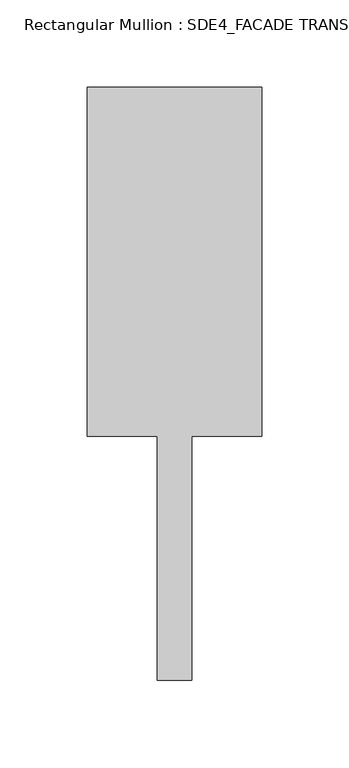
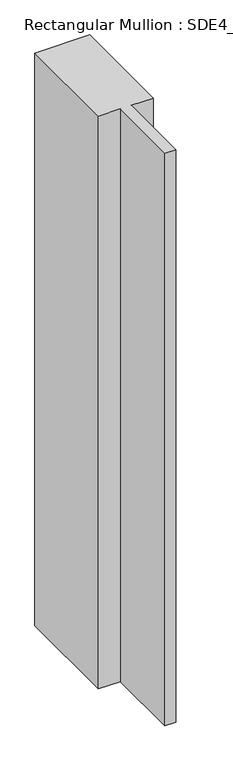
"""IFC4 building model written with IfcOpenShell, lengths in millimetres: member geometry, Rectangular Mullion : SDE4_FACADE TRANSOM TYPE 1."""

import ifcopenshell
import ifcopenshell.guid

model = None  # the IFC model being written
_history = None  # IfcOwnerHistory: only IFC2X3 demands one
_inside = {}  # id of a spatial element -> (the spatial element, [elements in it])
_under = {}  # id of a project, library or spatial element -> (it, [spatial elements below it])
_declared = {}  # id of a project -> (the project, [libraries it declares])
_typed = {}  # id of a type object -> (the type object, [elements of that type])
_made_of = {}  # id of a material, layer set ... -> (it, [elements and type objects made of it])


def new_model(schema):
    """Start an empty IFC model of exactly this schema.

    Asked for "IFC4X3", IfcOpenShell would pick the latest addendum, in which some entities
    have other attributes; the version numbers below select the first issue.
    IFC2X3 requires an IfcOwnerHistory on every rooted entity: one is made here for all.
    """
    global model, _history
    if schema == "IFC4X3":
        model = ifcopenshell.file(schema_version=(4, 3, 0, 0))
    else:
        model = ifcopenshell.file(schema=schema)
    _inside.clear()
    _under.clear()
    _declared.clear()
    _typed.clear()
    _made_of.clear()
    _history = None
    if model.schema == "IFC2X3":
        org = make("IfcOrganization", Name="unknown")
        user = make(
            "IfcPersonAndOrganization",
            ThePerson=make("IfcPerson", FamilyName="unknown"),
            TheOrganization=org,
        )
        app = make(
            "IfcApplication",
            ApplicationDeveloper=org,
            Version="unknown",
            ApplicationFullName="unknown",
            ApplicationIdentifier="unknown",
        )
        _history = make(
            "IfcOwnerHistory",
            OwningUser=user,
            OwningApplication=app,
            ChangeAction="ADDED",
            CreationDate=0,
        )
    return model


def make(cls, **values):
    """One entity of the class cls with the attributes given. An attribute that is None is left unset."""
    return model.create_entity(
        cls, **{name: value for name, value in values.items() if value is not None}
    )


def rooted(cls, **values):
    """An entity with a GlobalId (a new one), such as an element, a storey or a relation."""
    return make(cls, GlobalId=ifcopenshell.guid.new(), OwnerHistory=_history, **values)


def si_unit(unit_type, name, prefix=None):
    """IfcSIUnit, for example si_unit("LENGTHUNIT", "METRE", prefix="MILLI")."""
    return make("IfcSIUnit", UnitType=unit_type, Prefix=prefix, Name=name)


def assignment(units):
    """IfcUnitAssignment: the units of a project."""
    return None if units is None else make("IfcUnitAssignment", Units=units)


def point(xyz):
    """IfcCartesianPoint."""
    return None if xyz is None else make("IfcCartesianPoint", Coordinates=xyz)


def direction(xyz):
    """IfcDirection."""
    return None if xyz is None else make("IfcDirection", DirectionRatios=xyz)


def frame(location, z_axis=None, x_axis=None):
    """IfcAxis2Placement3D, a coordinate frame: its origin and axes. An axis left out is left unset."""
    return make(
        "IfcAxis2Placement3D",
        Location=point(location),
        Axis=direction(z_axis),
        RefDirection=direction(x_axis),
    )


def origin():
    """The frame at (0, 0, 0) with its axes left unset."""
    return frame((0.0, 0.0, 0.0))


def place(relative_to, where):
    """IfcLocalPlacement: puts the frame where relative to a parent placement (None: the world)."""
    return make(
        "IfcLocalPlacement", PlacementRelTo=relative_to, RelativePlacement=where
    )


def context(
    kind, dimensions, precision=None, world=None, true_north=None, identifier=None
):
    """IfcGeometricRepresentationContext, for example the 3D "Model" context."""
    return make(
        "IfcGeometricRepresentationContext",
        ContextIdentifier=identifier,
        ContextType=kind,
        CoordinateSpaceDimension=dimensions,
        Precision=precision,
        WorldCoordinateSystem=world,
        TrueNorth=true_north,
    )


def project(units=None, contexts=None):
    """IfcProject with its units and contexts."""
    return rooted(
        "IfcProject",
        Name="project",
        RepresentationContexts=contexts,
        UnitsInContext=assignment(units),
    )


def spatial(cls, under=None, at=None, **own):
    """A site, building, storey or space (cls), placed at a placement, below another one or the project."""
    s = rooted(cls, ObjectPlacement=at, **own)
    if under is not None:
        _under.setdefault(under.id(), (under, []))[1].append(s)
    return s


def polyline(points):
    """IfcPolyline through the points."""
    return make("IfcPolyline", Points=[point(p) for p in points])


def outline(outer, holes=None, kind="AREA"):
    """IfcArbitraryClosedProfileDef: a profile drawn as a closed curve; with holes, ...WithVoids."""
    if holes is None:
        return make("IfcArbitraryClosedProfileDef", ProfileType=kind, OuterCurve=outer)
    return make(
        "IfcArbitraryProfileDefWithVoids",
        ProfileType=kind,
        OuterCurve=outer,
        InnerCurves=holes,
    )


def extrude(swept, where, along, depth):
    """IfcExtrudedAreaSolid: the profile swept, set in the frame where, extruded along a direction by depth."""
    return make(
        "IfcExtrudedAreaSolid",
        SweptArea=swept,
        Position=where,
        ExtrudedDirection=direction(along),
        Depth=depth,
    )


def shape(context_of_items, identifier, shape_type, items):
    """IfcShapeRepresentation: the items that make up one representation, for example the "Body"."""
    return make(
        "IfcShapeRepresentation",
        ContextOfItems=context_of_items,
        RepresentationIdentifier=identifier,
        RepresentationType=shape_type,
        Items=items,
    )


def source(mapping_origin, context_of_items, identifier, shape_type, items):
    """IfcRepresentationMap: a shape defined once, which mapped items show again and again."""
    return make(
        "IfcRepresentationMap",
        MappingOrigin=mapping_origin,
        MappedRepresentation=shape(context_of_items, identifier, shape_type, items),
    )


def transform(
    local_origin,
    x_axis=None,
    y_axis=None,
    z_axis=None,
    scale=None,
    scale2=None,
    scale3=None,
    uniform=True,
):
    """IfcCartesianTransformationOperator3D, or its non-uniform kind. x_axis, y_axis, z_axis: its Axis1, 2, 3."""
    if uniform:
        return make(
            "IfcCartesianTransformationOperator3D",
            Axis1=direction(x_axis),
            Axis2=direction(y_axis),
            LocalOrigin=point(local_origin),
            Scale=scale,
            Axis3=direction(z_axis),
        )
    return make(
        "IfcCartesianTransformationOperator3DnonUniform",
        Axis1=direction(x_axis),
        Axis2=direction(y_axis),
        LocalOrigin=point(local_origin),
        Scale=scale,
        Axis3=direction(z_axis),
        Scale2=scale2,
        Scale3=scale3,
    )


def mapped(mapping_source, mapping_target):
    """IfcMappedItem: shows the shape of a source again, moved by a transform."""
    return make(
        "IfcMappedItem", MappingSource=mapping_source, MappingTarget=mapping_target
    )


def made_of(thing, what):
    """Note that an element or type object is made of a material, layer set ...; save() writes the relation."""
    if what is not None:
        _made_of.setdefault(what.id(), (what, []))[1].append(thing)
    return thing


def element(
    cls,
    number,
    at=None,
    inside=None,
    cuts=None,
    type_object=None,
    material=None,
    context=None,
    identifier="Body",
    shape_type=None,
    held_by="IfcProductDefinitionShape",
    body=None,
    shapes=None,
    **own,
):
    """One element of the class cls, such as IfcWall. Its Tag is "e" and its number.

    at: its placement. inside: the storey or other place that contains it. cuts: it is an
    opening in that element (IfcRelVoidsElement). A single representation is given by context,
    identifier, shape_type and body (its items); several are given by shapes. held_by: the class
    of the entity that holds the representations. save() writes the other relations.
    """
    e = rooted(cls, Tag="e%d" % number, ObjectPlacement=at, **own)
    if body is not None:
        shapes = [shape(context, identifier, shape_type, body)]
    if shapes is not None:
        e.Representation = make(held_by, Representations=shapes)
    if inside is not None:
        _inside.setdefault(inside.id(), (inside, []))[1].append(e)
    if cuts is not None:
        rooted(
            "IfcRelVoidsElement", RelatingBuildingElement=cuts, RelatedOpeningElement=e
        )
    if type_object is not None:
        _typed.setdefault(type_object.id(), (type_object, []))[1].append(e)
    return made_of(e, material)


def aggregate(whole, parts):
    """IfcRelAggregates: a whole, such as a stair, and the parts it consists of."""
    return rooted("IfcRelAggregates", RelatingObject=whole, RelatedObjects=parts)


def save(model, path):
    """Write the relations noted so far, then the file.

    IfcRelAggregates (storeys below a building ...), IfcRelContainedInSpatialStructure (elements
    in a storey), IfcRelDefinesByType, IfcRelAssociatesMaterial and IfcRelDeclares: one each for
    every whole, place, type object, material and project.
    """
    for whole, parts in _under.values():
        aggregate(whole, parts)
    for where, things in _inside.values():
        rooted(
            "IfcRelContainedInSpatialStructure",
            RelatedElements=things,
            RelatingStructure=where,
        )
    for kind, things in _typed.values():
        rooted("IfcRelDefinesByType", RelatedObjects=things, RelatingType=kind)
    for what, things in _made_of.values():
        rooted("IfcRelAssociatesMaterial", RelatedObjects=things, RelatingMaterial=what)
    for by, libraries in _declared.values():
        rooted("IfcRelDeclares", RelatingContext=by, RelatedDefinitions=libraries)
    model.write(path)


def rectangular_mullion_sde4_facade_transom_type_1_68cbf1c2(model_context):
    return source(origin(), model_context, "Body", "SweptSolid", [
        extrude(outline(polyline([(50.0, 132.5), (50.0, -67.5), (10.0, -67.5), (10.0, -207.5), (-10.0, -207.5), (-10.0, -67.5), (-50.0, -67.5), (-50.0, 132.5), (50.0, 132.5)])), frame((0.0, 0.0, -1100.0), z_axis=(0.0, 0.0, 1.0), x_axis=(1.0, 0.0, 0.0)), (0.0, 0.0, 1.0), 1100.0),
    ])


if __name__ == "__main__":
    model = new_model("IFC4")
    model_context = context("Model", 3, world=origin())
    ifc_project = project(units=[si_unit("LENGTHUNIT", "METRE", prefix="MILLI")], contexts=[model_context])
    site = spatial("IfcSite", under=ifc_project)
    building = spatial("IfcBuilding", under=site)
    placement = place(None, origin())
    rectangular_mullion_sde4_facade_transom_type_1_shape = rectangular_mullion_sde4_facade_transom_type_1_68cbf1c2(model_context)
    element("IfcMember", 1, ObjectType="Rectangular Mullion : SDE4_FACADE TRANSOM TYPE 1", at=placement, inside=building, context=model_context, shape_type="MappedRepresentation", body=[
        mapped(rectangular_mullion_sde4_facade_transom_type_1_shape, transform((0.0, 0.0, 0.0), x_axis=(1.0, 0.0, 0.0), y_axis=(0.0, 1.0, 0.0), z_axis=(0.0, 0.0, 1.0))),
    ])
    save(model, "model.ifc")

# Revit data of these elements
# Type "Rectangular Mullion : SDE4_FACADE TRANSOM TYPE 1"
#   built-in parameter 1007322 = 1.11549 (stored number, unit not read)
#   built-in parameter 1007321 = 0.164042 (stored number, unit not read)
#   built-in parameter 1007320 = 0.164042 (stored number, unit not read)
